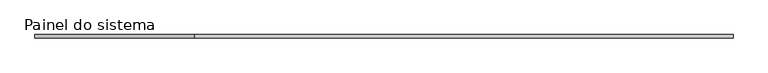
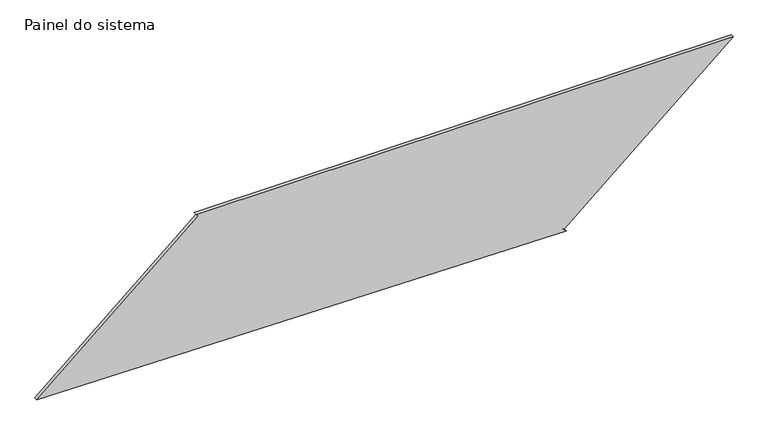
"""IFC4 building model written with IfcOpenShell, lengths in millimetres: plate geometry, Painel do sistema : Envidraçado."""

from ifc_helpers import new_model, si_unit, frame, origin, place, context, project, spatial, polyline, outline, extrude, source, transform, mapped, element, save


def painel_do_sistema_f9066246(model_context):
    return source(origin(), model_context, "Body", "SweptSolid", [
        extrude(outline(polyline([(0.0, 1323.4084222), (19.0100862, 1307.1721472), (1074.8206644, 2543.3577982), (1074.8206644, -1379.3845646), (1055.8105782, -1363.1482897), (47.8085175, -2543.3577982), (0.0, 1323.4084222)])), frame((0.0, 24.5, 0.0), z_axis=(0.0, 1.0, 0.0), x_axis=(0.0, 0.0, 1.0)), (0.0, 0.0, 1.0), 25.0),
    ])


if __name__ == "__main__":
    model = new_model("IFC4")
    model_context = context("Model", 3, world=origin())
    ifc_project = project(units=[si_unit("LENGTHUNIT", "METRE", prefix="MILLI")], contexts=[model_context])
    site = spatial("IfcSite", under=ifc_project)
    building = spatial("IfcBuilding", under=site)
    placement = place(None, origin())
    painel_do_sistema_shape = painel_do_sistema_f9066246(model_context)
    element("IfcPlate", 1, ObjectType="Painel do sistema : Envidraçado", at=placement, inside=building, context=model_context, shape_type="MappedRepresentation", body=[
        mapped(painel_do_sistema_shape, transform((0.0, 0.0, 0.0), x_axis=(1.0, 0.0, 0.0), y_axis=(0.0, 1.0, 0.0), z_axis=(0.0, 0.0, 1.0))),
    ])
    save(model, "model.ifc")

# Revit data of these elements
# Type "Painel do sistema : Envidraçado"
#   Construction Type Id = "GSP4R"
#   Analytic Construction = "Vidraça única Pilkington 1/8 pol"
#   Visual Light Transmittance = 0.9
#   Solar Heat Gain Coefficient = 0.86
#   Heat Transfer Coefficient (U) = 6.7069 W/(m²·K)
# Element 1 (IfcPlate, "Painel do sistema : Envidraçado")
#   Materials on its faces: "Vidro"
# Materials
#   "Vidro": class "Vidro", colour RGB 0 128 192, transparency 0.9, Description = "Vidro de sílica", Cost = 0
